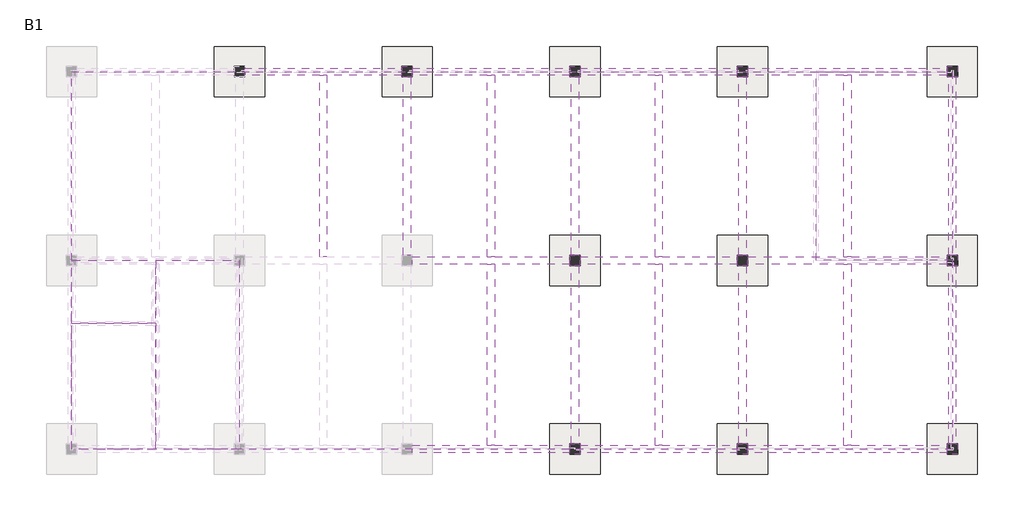
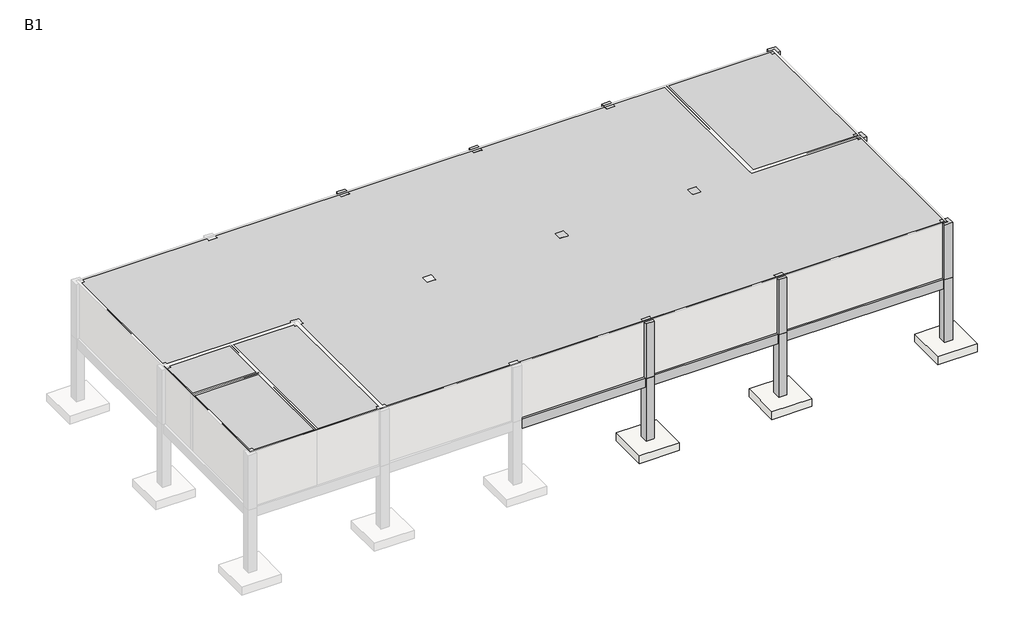
# One storey, part 2 of 2: 24 beams, 21 columns, 11 slabs, 5 proxies.
"""IFC4 building model written with IfcOpenShell, lengths in millimetres."""

import ifcopenshell
import ifcopenshell.guid

model = None  # the IFC model being written
_history = None  # IfcOwnerHistory: only IFC2X3 demands one
_inside = {}  # id of a spatial element -> (the spatial element, [elements in it])
_under = {}  # id of a project, library or spatial element -> (it, [spatial elements below it])
_declared = {}  # id of a project -> (the project, [libraries it declares])
_typed = {}  # id of a type object -> (the type object, [elements of that type])
_made_of = {}  # id of a material, layer set ... -> (it, [elements and type objects made of it])


def new_model(schema):
    """Start an empty IFC model of exactly this schema.

    Asked for "IFC4X3", IfcOpenShell would pick the latest addendum, in which some entities
    have other attributes; the version numbers below select the first issue.
    IFC2X3 requires an IfcOwnerHistory on every rooted entity: one is made here for all.
    """
    global model, _history
    if schema == "IFC4X3":
        model = ifcopenshell.file(schema_version=(4, 3, 0, 0))
    else:
        model = ifcopenshell.file(schema=schema)
    _inside.clear()
    _under.clear()
    _declared.clear()
    _typed.clear()
    _made_of.clear()
    _history = None
    if model.schema == "IFC2X3":
        org = make("IfcOrganization", Name="unknown")
        user = make(
            "IfcPersonAndOrganization",
            ThePerson=make("IfcPerson", FamilyName="unknown"),
            TheOrganization=org,
        )
        app = make(
            "IfcApplication",
            ApplicationDeveloper=org,
            Version="unknown",
            ApplicationFullName="unknown",
            ApplicationIdentifier="unknown",
        )
        _history = make(
            "IfcOwnerHistory",
            OwningUser=user,
            OwningApplication=app,
            ChangeAction="ADDED",
            CreationDate=0,
        )
    return model


def make(cls, **values):
    """One entity of the class cls with the attributes given. An attribute that is None is left unset."""
    return model.create_entity(
        cls, **{name: value for name, value in values.items() if value is not None}
    )


def rooted(cls, **values):
    """An entity with a GlobalId (a new one), such as an element, a storey or a relation."""
    return make(cls, GlobalId=ifcopenshell.guid.new(), OwnerHistory=_history, **values)


def si_unit(unit_type, name, prefix=None):
    """IfcSIUnit, for example si_unit("LENGTHUNIT", "METRE", prefix="MILLI")."""
    return make("IfcSIUnit", UnitType=unit_type, Prefix=prefix, Name=name)


def assignment(units):
    """IfcUnitAssignment: the units of a project."""
    return None if units is None else make("IfcUnitAssignment", Units=units)


def point(xyz):
    """IfcCartesianPoint."""
    return None if xyz is None else make("IfcCartesianPoint", Coordinates=xyz)


def direction(xyz):
    """IfcDirection."""
    return None if xyz is None else make("IfcDirection", DirectionRatios=xyz)


def frame(location, z_axis=None, x_axis=None):
    """IfcAxis2Placement3D, a coordinate frame: its origin and axes. An axis left out is left unset."""
    return make(
        "IfcAxis2Placement3D",
        Location=point(location),
        Axis=direction(z_axis),
        RefDirection=direction(x_axis),
    )


def origin():
    """The frame at (0, 0, 0) with its axes left unset."""
    return frame((0.0, 0.0, 0.0))


def origin_with_axes():
    """The frame at (0, 0, 0) with the z axis (0, 0, 1) and the x axis (1, 0, 0) written out."""
    return frame((0.0, 0.0, 0.0), z_axis=(0.0, 0.0, 1.0), x_axis=(1.0, 0.0, 0.0))


def place(relative_to, where):
    """IfcLocalPlacement: puts the frame where relative to a parent placement (None: the world)."""
    return make(
        "IfcLocalPlacement", PlacementRelTo=relative_to, RelativePlacement=where
    )


def context(
    kind, dimensions, precision=None, world=None, true_north=None, identifier=None
):
    """IfcGeometricRepresentationContext, for example the 3D "Model" context."""
    return make(
        "IfcGeometricRepresentationContext",
        ContextIdentifier=identifier,
        ContextType=kind,
        CoordinateSpaceDimension=dimensions,
        Precision=precision,
        WorldCoordinateSystem=world,
        TrueNorth=true_north,
    )


def project(units=None, contexts=None):
    """IfcProject with its units and contexts."""
    return rooted(
        "IfcProject",
        Name="project",
        RepresentationContexts=contexts,
        UnitsInContext=assignment(units),
    )


def spatial(cls, under=None, at=None, **own):
    """A site, building, storey or space (cls), placed at a placement, below another one or the project."""
    s = rooted(cls, ObjectPlacement=at, **own)
    if under is not None:
        _under.setdefault(under.id(), (under, []))[1].append(s)
    return s


def polyline(points):
    """IfcPolyline through the points."""
    return make("IfcPolyline", Points=[point(p) for p in points])


def outline(outer, holes=None, kind="AREA"):
    """IfcArbitraryClosedProfileDef: a profile drawn as a closed curve; with holes, ...WithVoids."""
    if holes is None:
        return make("IfcArbitraryClosedProfileDef", ProfileType=kind, OuterCurve=outer)
    return make(
        "IfcArbitraryProfileDefWithVoids",
        ProfileType=kind,
        OuterCurve=outer,
        InnerCurves=holes,
    )


def extrude(swept, where, along, depth):
    """IfcExtrudedAreaSolid: the profile swept, set in the frame where, extruded along a direction by depth."""
    return make(
        "IfcExtrudedAreaSolid",
        SweptArea=swept,
        Position=where,
        ExtrudedDirection=direction(along),
        Depth=depth,
    )


def faces_of(points, faces, orient=None, outer=None):
    """IfcFace entities. A face is a list of loops; a loop is a list of indices into points, from 0.

    orient and outer hold one flag for each loop. By default every Orientation is true, the
    first loop of a face is its IfcFaceOuterBound and the others are IfcFaceBound.
    """
    made = []
    for i, loops in enumerate(faces):
        bounds = []
        for j, loop in enumerate(loops):
            is_outer = j == 0 if outer is None else outer[i][j]
            bounds.append(
                make(
                    "IfcFaceOuterBound" if is_outer else "IfcFaceBound",
                    Bound=make("IfcPolyLoop", Polygon=[points[k] for k in loop]),
                    Orientation=True if orient is None else orient[i][j],
                )
            )
        made.append(make("IfcFace", Bounds=bounds))
    return made


def faceted_brep(points, faces, orient=None, outer=None, voids=None):
    """IfcFacetedBrep: a solid bounded by flat faces; with voids (closed shells), ...WithVoids."""
    shared = [point(p) for p in points]
    hull = make("IfcClosedShell", CfsFaces=faces_of(shared, faces, orient, outer))
    if voids is None:
        return make("IfcFacetedBrep", Outer=hull)
    return make(
        "IfcFacetedBrepWithVoids",
        Outer=hull,
        Voids=[
            make(cls, CfsFaces=faces_of(shared, fs, o, b)) for cls, fs, o, b in voids
        ],
    )


def shape(context_of_items, identifier, shape_type, items):
    """IfcShapeRepresentation: the items that make up one representation, for example the "Body"."""
    return make(
        "IfcShapeRepresentation",
        ContextOfItems=context_of_items,
        RepresentationIdentifier=identifier,
        RepresentationType=shape_type,
        Items=items,
    )


def source(mapping_origin, context_of_items, identifier, shape_type, items):
    """IfcRepresentationMap: a shape defined once, which mapped items show again and again."""
    return make(
        "IfcRepresentationMap",
        MappingOrigin=mapping_origin,
        MappedRepresentation=shape(context_of_items, identifier, shape_type, items),
    )


def transform(
    local_origin,
    x_axis=None,
    y_axis=None,
    z_axis=None,
    scale=None,
    scale2=None,
    scale3=None,
    uniform=True,
):
    """IfcCartesianTransformationOperator3D, or its non-uniform kind. x_axis, y_axis, z_axis: its Axis1, 2, 3."""
    if uniform:
        return make(
            "IfcCartesianTransformationOperator3D",
            Axis1=direction(x_axis),
            Axis2=direction(y_axis),
            LocalOrigin=point(local_origin),
            Scale=scale,
            Axis3=direction(z_axis),
        )
    return make(
        "IfcCartesianTransformationOperator3DnonUniform",
        Axis1=direction(x_axis),
        Axis2=direction(y_axis),
        LocalOrigin=point(local_origin),
        Scale=scale,
        Axis3=direction(z_axis),
        Scale2=scale2,
        Scale3=scale3,
    )


def mapped(mapping_source, mapping_target):
    """IfcMappedItem: shows the shape of a source again, moved by a transform."""
    return make(
        "IfcMappedItem", MappingSource=mapping_source, MappingTarget=mapping_target
    )


def made_of(thing, what):
    """Note that an element or type object is made of a material, layer set ...; save() writes the relation."""
    if what is not None:
        _made_of.setdefault(what.id(), (what, []))[1].append(thing)
    return thing


def element(
    cls,
    number,
    at=None,
    inside=None,
    cuts=None,
    type_object=None,
    material=None,
    context=None,
    identifier="Body",
    shape_type=None,
    held_by="IfcProductDefinitionShape",
    body=None,
    shapes=None,
    **own,
):
    """One element of the class cls, such as IfcWall. Its Tag is "e" and its number.

    at: its placement. inside: the storey or other place that contains it. cuts: it is an
    opening in that element (IfcRelVoidsElement). A single representation is given by context,
    identifier, shape_type and body (its items); several are given by shapes. held_by: the class
    of the entity that holds the representations. save() writes the other relations.
    """
    e = rooted(cls, Tag="e%d" % number, ObjectPlacement=at, **own)
    if body is not None:
        shapes = [shape(context, identifier, shape_type, body)]
    if shapes is not None:
        e.Representation = make(held_by, Representations=shapes)
    if inside is not None:
        _inside.setdefault(inside.id(), (inside, []))[1].append(e)
    if cuts is not None:
        rooted(
            "IfcRelVoidsElement", RelatingBuildingElement=cuts, RelatedOpeningElement=e
        )
    if type_object is not None:
        _typed.setdefault(type_object.id(), (type_object, []))[1].append(e)
    return made_of(e, material)


def aggregate(whole, parts):
    """IfcRelAggregates: a whole, such as a stair, and the parts it consists of."""
    return rooted("IfcRelAggregates", RelatingObject=whole, RelatedObjects=parts)


def save(model, path):
    """Write the relations noted so far, then the file.

    IfcRelAggregates (storeys below a building ...), IfcRelContainedInSpatialStructure (elements
    in a storey), IfcRelDefinesByType, IfcRelAssociatesMaterial and IfcRelDeclares: one each for
    every whole, place, type object, material and project.
    """
    for whole, parts in _under.values():
        aggregate(whole, parts)
    for where, things in _inside.values():
        rooted(
            "IfcRelContainedInSpatialStructure",
            RelatedElements=things,
            RelatingStructure=where,
        )
    for kind, things in _typed.values():
        rooted("IfcRelDefinesByType", RelatedObjects=things, RelatingType=kind)
    for what, things in _made_of.values():
        rooted("IfcRelAssociatesMaterial", RelatedObjects=things, RelatingMaterial=what)
    for by, libraries in _declared.values():
        rooted("IfcRelDeclares", RelatingContext=by, RelatedDefinitions=libraries)
    model.write(path)


def generic_models_bb515c93(model_context):
    return source(origin(), model_context, "Body", "SweptSolid", [
        extrude(outline(polyline([(9000.0, 21000.0), (9000.0, -21000.0), (-9000.0, -21000.0), (-9000.0, 21000.0), (9000.0, 21000.0)])), origin_with_axes(), (0.0, 0.0, 1.0), 3500.0),
    ])


def generic_models_5926095e(model_context):
    return source(origin(), model_context, "Body", "SweptSolid", [
        extrude(outline(polyline([(3250.0, 4500.0), (3250.0, -4500.0), (-3250.0, -4500.0), (-3250.0, 4500.0), (3250.0, 4500.0)])), origin_with_axes(), (0.0, 0.0, 1.0), 3500.0),
    ])


def generic_models_0b067365(model_context):
    return source(origin(), model_context, "Body", "SweptSolid", [
        extrude(outline(polyline([(2000.0, 4500.0), (2000.0, -4500.0), (-2000.0, -4500.0), (-2000.0, 4500.0), (2000.0, 4500.0)])), origin_with_axes(), (0.0, 0.0, 1.0), 3500.0),
    ])


def generic_models_4c644d41(model_context):
    return source(origin(), model_context, "Body", "SweptSolid", [
        extrude(outline(polyline([(2000.0, 1500.0), (2000.0, -1500.0), (-2000.0, -1500.0), (-2000.0, 1500.0), (2000.0, 1500.0)])), origin_with_axes(), (0.0, 0.0, 1.0), 3500.0),
    ])


def generic_models_c89eb543(model_context):
    return source(origin(), model_context, "Body", "SweptSolid", [
        extrude(outline(polyline([(2000.0, 3000.0), (2000.0, -3000.0), (-2000.0, -3000.0), (-2000.0, 3000.0), (2000.0, 3000.0)])), origin_with_axes(), (0.0, 0.0, 1.0), 3500.0),
    ])


def ft112_footing_rectangular_ft112_2400x2400x500_5fe39465(model_context):
    return source(origin(), model_context, "Body", "SweptSolid", [
        extrude(outline(polyline([(1200.0, 1200.0), (1200.0, -1200.0), (-1200.0, -1200.0), (-1200.0, 1200.0), (1200.0, 1200.0)])), frame((0.0, 0.0, -500.0), z_axis=(0.0, 0.0, 1.0), x_axis=(1.0, 0.0, 0.0)), (0.0, 0.0, 1.0), 500.0),
    ])


model = new_model("IFC4")

# Units and contexts
model_context = context("Model", 3, world=origin())
ifc_project = project(units=[si_unit("LENGTHUNIT", "METRE", prefix="MILLI")], contexts=[model_context])

# Site, building, storey
site = spatial("IfcSite", under=ifc_project)
building = spatial("IfcBuilding", under=site)
storey = spatial("IfcBuildingStorey", under=building, Name="B1", Elevation=-4000.0)

# Beams
placement = place(None, origin())
element("IfcBeam", 1, ObjectType="Concrete-Rectangular-Beam : BM111_400x500_RG1", at=placement, inside=storey, context=model_context, shape_type="SweptSolid", body=[
    extrude(outline(polyline([(57634.6521483, 173098.8614395), (57284.6521483, 173098.8614395), (57284.6521483, 181748.8614395), (57634.6521483, 181748.8614395), (57634.6521483, 173098.8614395)])), frame((0.0, 0.0, -600.0), z_axis=(0.0, 0.0, 1.0), x_axis=(1.0, 0.0, 0.0)), (0.0, 0.0, 1.0), 600.0),
])
element("IfcBeam", 2, ObjectType="Concrete-Rectangular-Beam : BM111_400x500_RG1", at=placement, inside=storey, context=model_context, shape_type="SweptSolid", body=[
    extrude(outline(polyline([(65634.6521483, 173098.8614395), (65284.6521483, 173098.8614395), (65284.6521483, 181748.8614395), (65634.6521483, 181748.8614395), (65634.6521483, 173098.8614395)])), frame((0.0, 0.0, -600.0), z_axis=(0.0, 0.0, 1.0), x_axis=(1.0, 0.0, 0.0)), (0.0, 0.0, 1.0), 600.0),
])
element("IfcBeam", 3, ObjectType="Concrete-Rectangular-Beam : BM111_400x500_RG1", at=placement, inside=storey, context=model_context, shape_type="SweptSolid", body=[
    extrude(outline(polyline([(65284.6521483, 172748.8614395), (65634.6521483, 172748.8614395), (65634.6521483, 164098.8614395), (65284.6521483, 164098.8614395), (65284.6521483, 172748.8614395)])), frame((0.0, 0.0, -600.0), z_axis=(0.0, 0.0, 1.0), x_axis=(1.0, 0.0, 0.0)), (0.0, 0.0, 1.0), 600.0),
])
element("IfcBeam", 4, ObjectType="Concrete-Rectangular-Beam : BM111_400x500_RG1", at=placement, inside=storey, context=model_context, shape_type="SweptSolid", body=[
    extrude(outline(polyline([(73634.6521483, 173098.8614395), (73284.6521483, 173098.8614395), (73284.6521483, 181748.8614395), (73634.6521483, 181748.8614395), (73634.6521483, 173098.8614395)])), frame((0.0, 0.0, -600.0), z_axis=(0.0, 0.0, 1.0), x_axis=(1.0, 0.0, 0.0)), (0.0, 0.0, 1.0), 600.0),
])
element("IfcBeam", 5, ObjectType="Concrete-Rectangular-Beam : BM111_400x500_RG1", at=placement, inside=storey, context=model_context, shape_type="SweptSolid", body=[
    extrude(outline(polyline([(73284.6521483, 172748.8614395), (73634.6521483, 172748.8614395), (73634.6521483, 164098.8614395), (73284.6521483, 164098.8614395), (73284.6521483, 172748.8614395)])), frame((0.0, 0.0, -600.0), z_axis=(0.0, 0.0, 1.0), x_axis=(1.0, 0.0, 0.0)), (0.0, 0.0, 1.0), 600.0),
])
element("IfcBeam", 6, ObjectType="Concrete-Rectangular-Beam : BM111_400x500_RG1", at=placement, inside=storey, context=model_context, shape_type="SweptSolid", body=[
    extrude(outline(polyline([(82634.6521483, 173098.8614395), (82284.6521483, 173098.8614395), (82284.6521483, 181748.8614395), (82634.6521483, 181748.8614395), (82634.6521483, 173098.8614395)])), frame((0.0, 0.0, -600.0), z_axis=(0.0, 0.0, 1.0), x_axis=(1.0, 0.0, 0.0)), (0.0, 0.0, 1.0), 600.0),
])
element("IfcBeam", 7, ObjectType="Concrete-Rectangular-Beam : BM111_400x500_RG1", at=placement, inside=storey, context=model_context, shape_type="SweptSolid", body=[
    extrude(outline(polyline([(82284.6521483, 172748.8614395), (82634.6521483, 172748.8614395), (82634.6521483, 164098.8614395), (82284.6521483, 164098.8614395), (82284.6521483, 172748.8614395)])), frame((0.0, 0.0, -600.0), z_axis=(0.0, 0.0, 1.0), x_axis=(1.0, 0.0, 0.0)), (0.0, 0.0, 1.0), 600.0),
])
element("IfcBeam", 8, ObjectType="Concrete-Rectangular-Beam : BM111_400x500_RG1", at=placement, inside=storey, context=model_context, shape_type="Brep", body=[
    faceted_brep([(53709.6521483, 182098.8614395, 0.0), (53709.6521483, 181748.8614395, 0.0), (57284.6521483, 181748.8614395, 0.0), (57634.6521483, 181748.8614395, 0.0), (61209.6521483, 181748.8614395, 0.0), (61209.6521483, 182098.8614395, 0.0), (53709.6521483, 181748.8614395, -600.0), (57284.6521483, 181748.8614395, -600.0), (57634.6521483, 181748.8614395, -600.0), (61209.6521483, 181748.8614395, -600.0), (53709.6521483, 182098.8614395, -600.0), (61209.6521483, 182098.8614395, -600.0)], [[[0, 1, 2, 3, 4, 5]], [[1, 6, 7, 8, 9, 4, 3, 2]], [[6, 10, 11, 9, 8, 7]], [[10, 0, 5, 11]], [[1, 0, 10, 6]], [[5, 4, 9, 11]]]),
])
element("IfcBeam", 9, ObjectType="Concrete-Rectangular-Beam : BM111_400x500_RG1", at=placement, inside=storey, context=model_context, shape_type="Brep", body=[
    faceted_brep([(61709.6521483, 182098.8614395, 0.0), (61709.6521483, 181748.8614395, 0.0), (65284.6521483, 181748.8614395, 0.0), (65634.6521483, 181748.8614395, 0.0), (69209.6521483, 181748.8614395, 0.0), (69209.6521483, 182098.8614395, 0.0), (61709.6521483, 181748.8614395, -600.0), (65284.6521483, 181748.8614395, -600.0), (65634.6521483, 181748.8614395, -600.0), (69209.6521483, 181748.8614395, -600.0), (61709.6521483, 182098.8614395, -600.0), (69209.6521483, 182098.8614395, -600.0)], [[[0, 1, 2, 3, 4, 5]], [[1, 6, 7, 8, 9, 4, 3, 2]], [[6, 10, 11, 9, 8, 7]], [[10, 0, 5, 11]], [[1, 0, 10, 6]], [[5, 4, 9, 11]]]),
])
element("IfcBeam", 10, ObjectType="Concrete-Rectangular-Beam : BM111_400x500_RG1", at=placement, inside=storey, context=model_context, shape_type="Brep", body=[
    faceted_brep([(69709.6521483, 182098.8614395, 0.0), (69709.6521483, 181748.8614395, 0.0), (73284.6521483, 181748.8614395, 0.0), (73634.6521483, 181748.8614395, 0.0), (77209.6521483, 181748.8614395, 0.0), (77209.6521483, 182098.8614395, 0.0), (69709.6521483, 181748.8614395, -600.0), (73284.6521483, 181748.8614395, -600.0), (73634.6521483, 181748.8614395, -600.0), (77209.6521483, 181748.8614395, -600.0), (69709.6521483, 182098.8614395, -600.0), (77209.6521483, 182098.8614395, -600.0)], [[[0, 1, 2, 3, 4, 5]], [[1, 6, 7, 8, 9, 4, 3, 2]], [[6, 10, 11, 9, 8, 7]], [[10, 0, 5, 11]], [[1, 0, 10, 6]], [[5, 4, 9, 11]]]),
])
element("IfcBeam", 11, ObjectType="Concrete-Rectangular-Beam : BM111_400x500_RG1", at=placement, inside=storey, context=model_context, shape_type="Brep", body=[
    faceted_brep([(77709.6521483, 182098.8614395, 0.0), (77709.6521483, 181748.8614395, 0.0), (82284.6521483, 181748.8614395, 0.0), (82634.6521483, 181748.8614395, 0.0), (87209.6521483, 181748.8614395, 0.0), (87209.6521483, 182098.8614395, 0.0), (77709.6521483, 181748.8614395, -600.0), (82284.6521483, 181748.8614395, -600.0), (82634.6521483, 181748.8614395, -600.0), (87209.6521483, 181748.8614395, -600.0), (77709.6521483, 182098.8614395, -600.0), (87209.6521483, 182098.8614395, -600.0)], [[[0, 1, 2, 3, 4, 5]], [[1, 6, 7, 8, 9, 4, 3, 2]], [[6, 10, 11, 9, 8, 7]], [[10, 0, 5, 11]], [[1, 0, 10, 6]], [[5, 4, 9, 11]]]),
])
element("IfcBeam", 12, ObjectType="Concrete-Rectangular-Beam : BM111_400x500_RG1", at=placement, inside=storey, context=model_context, shape_type="Brep", body=[
    faceted_brep([(61709.6521483, 173098.8614395, 0.0), (61709.6521483, 172748.8614395, 0.0), (65284.6521483, 172748.8614395, 0.0), (65634.6521483, 172748.8614395, 0.0), (69209.6521483, 172748.8614395, 0.0), (69209.6521483, 173098.8614395, 0.0), (65634.6521483, 173098.8614395, 0.0), (65284.6521483, 173098.8614395, 0.0), (61709.6521483, 172748.8614395, -600.0), (65284.6521483, 172748.8614395, -600.0), (65634.6521483, 172748.8614395, -600.0), (69209.6521483, 172748.8614395, -600.0), (61709.6521483, 173098.8614395, -600.0), (65284.6521483, 173098.8614395, -600.0), (65634.6521483, 173098.8614395, -600.0), (69209.6521483, 173098.8614395, -600.0)], [[[0, 1, 2, 3, 4, 5, 6, 7]], [[1, 8, 9, 10, 11, 4, 3, 2]], [[8, 12, 13, 14, 15, 11, 10, 9]], [[12, 0, 7, 6, 5, 15, 14, 13]], [[1, 0, 12, 8]], [[5, 4, 11, 15]]]),
])
element("IfcBeam", 13, ObjectType="Concrete-Rectangular-Beam : BM111_400x500_RG1", at=placement, inside=storey, context=model_context, shape_type="Brep", body=[
    faceted_brep([(69709.6521483, 173098.8614395, 0.0), (69709.6521483, 172748.8614395, 0.0), (73284.6521483, 172748.8614395, 0.0), (73634.6521483, 172748.8614395, 0.0), (77209.6521483, 172748.8614395, 0.0), (77209.6521483, 173098.8614395, 0.0), (73634.6521483, 173098.8614395, 0.0), (73284.6521483, 173098.8614395, 0.0), (69709.6521483, 172748.8614395, -600.0), (73284.6521483, 172748.8614395, -600.0), (73634.6521483, 172748.8614395, -600.0), (77209.6521483, 172748.8614395, -600.0), (69709.6521483, 173098.8614395, -600.0), (73284.6521483, 173098.8614395, -600.0), (73634.6521483, 173098.8614395, -600.0), (77209.6521483, 173098.8614395, -600.0)], [[[0, 1, 2, 3, 4, 5, 6, 7]], [[1, 8, 9, 10, 11, 4, 3, 2]], [[8, 12, 13, 14, 15, 11, 10, 9]], [[12, 0, 7, 6, 5, 15, 14, 13]], [[1, 0, 12, 8]], [[5, 4, 11, 15]]]),
])
element("IfcBeam", 14, ObjectType="Concrete-Rectangular-Beam : BM111_400x500_RG1", at=placement, inside=storey, context=model_context, shape_type="Brep", body=[
    faceted_brep([(77709.6521483, 173098.8614395, 0.0), (77709.6521483, 172748.8614395, 0.0), (82284.6521483, 172748.8614395, 0.0), (82634.6521483, 172748.8614395, 0.0), (87209.6521483, 172748.8614395, 0.0), (87209.6521483, 173098.8614395, 0.0), (82634.6521483, 173098.8614395, 0.0), (82284.6521483, 173098.8614395, 0.0), (77709.6521483, 172748.8614395, -600.0), (82284.6521483, 172748.8614395, -600.0), (82634.6521483, 172748.8614395, -600.0), (87209.6521483, 172748.8614395, -600.0), (77709.6521483, 173098.8614395, -600.0), (82284.6521483, 173098.8614395, -600.0), (82634.6521483, 173098.8614395, -600.0), (87209.6521483, 173098.8614395, -600.0)], [[[0, 1, 2, 3, 4, 5, 6, 7]], [[1, 8, 9, 10, 11, 4, 3, 2]], [[8, 12, 13, 14, 15, 11, 10, 9]], [[12, 0, 7, 6, 5, 15, 14, 13]], [[1, 0, 12, 8]], [[5, 4, 11, 15]]]),
])
element("IfcBeam", 15, ObjectType="Concrete-Rectangular-Beam : BM111_400x500_RG1", at=placement, inside=storey, context=model_context, shape_type="Brep", body=[
    faceted_brep([(61709.6521483, 164098.8614395, 0.0), (61709.6521483, 163748.8614395, 0.0), (69209.6521483, 163748.8614395, 0.0), (69209.6521483, 164098.8614395, 0.0), (65634.6521483, 164098.8614395, 0.0), (65284.6521483, 164098.8614395, 0.0), (61709.6521483, 163748.8614395, -600.0), (69209.6521483, 163748.8614395, -600.0), (61709.6521483, 164098.8614395, -600.0), (65284.6521483, 164098.8614395, -600.0), (65634.6521483, 164098.8614395, -600.0), (69209.6521483, 164098.8614395, -600.0)], [[[0, 1, 2, 3, 4, 5]], [[1, 6, 7, 2]], [[6, 8, 9, 10, 11, 7]], [[8, 0, 5, 4, 3, 11, 10, 9]], [[1, 0, 8, 6]], [[3, 2, 7, 11]]]),
])
element("IfcBeam", 16, ObjectType="Concrete-Rectangular-Beam : BM111_400x500_RG1", at=placement, inside=storey, context=model_context, shape_type="Brep", body=[
    faceted_brep([(69709.6521483, 164098.8614395, 0.0), (69709.6521483, 163748.8614395, 0.0), (77209.6521483, 163748.8614395, 0.0), (77209.6521483, 164098.8614395, 0.0), (73634.6521483, 164098.8614395, 0.0), (73284.6521483, 164098.8614395, 0.0), (69709.6521483, 163748.8614395, -600.0), (77209.6521483, 163748.8614395, -600.0), (69709.6521483, 164098.8614395, -600.0), (73284.6521483, 164098.8614395, -600.0), (73634.6521483, 164098.8614395, -600.0), (77209.6521483, 164098.8614395, -600.0)], [[[0, 1, 2, 3, 4, 5]], [[1, 6, 7, 2]], [[6, 8, 9, 10, 11, 7]], [[8, 0, 5, 4, 3, 11, 10, 9]], [[1, 0, 8, 6]], [[3, 2, 7, 11]]]),
])
element("IfcBeam", 17, ObjectType="Concrete-Rectangular-Beam : BM111_400x500_RG1", at=placement, inside=storey, context=model_context, shape_type="Brep", body=[
    faceted_brep([(77709.6521483, 164098.8614395, 0.0), (77709.6521483, 163748.8614395, 0.0), (87209.6521483, 163748.8614395, 0.0), (87209.6521483, 164098.8614395, 0.0), (82634.6521483, 164098.8614395, 0.0), (82284.6521483, 164098.8614395, 0.0), (77709.6521483, 163748.8614395, -600.0), (87209.6521483, 163748.8614395, -600.0), (77709.6521483, 164098.8614395, -600.0), (82284.6521483, 164098.8614395, -600.0), (82634.6521483, 164098.8614395, -600.0), (87209.6521483, 164098.8614395, -600.0)], [[[0, 1, 2, 3, 4, 5]], [[1, 6, 7, 2]], [[6, 8, 9, 10, 11, 7]], [[8, 0, 5, 4, 3, 11, 10, 9]], [[1, 0, 8, 6]], [[3, 2, 7, 11]]]),
])
element("IfcBeam", 18, ObjectType="Concrete-Rectangular-Beam : BM111_400x500_RG1", at=placement, inside=storey, context=model_context, shape_type="SweptSolid", body=[
    extrude(outline(polyline([(61284.6521483, 181673.8614395), (61634.6521483, 181673.8614395), (61634.6521483, 173173.8614395), (61284.6521483, 173173.8614395), (61284.6521483, 181673.8614395)])), frame((0.0, 0.0, -600.0), z_axis=(0.0, 0.0, 1.0), x_axis=(1.0, 0.0, 0.0)), (0.0, 0.0, 1.0), 600.0),
])
element("IfcBeam", 19, ObjectType="Concrete-Rectangular-Beam : BM111_400x500_RG1", at=placement, inside=storey, context=model_context, shape_type="SweptSolid", body=[
    extrude(outline(polyline([(69284.6521483, 181673.8614395), (69634.6521483, 181673.8614395), (69634.6521483, 173173.8614395), (69284.6521483, 173173.8614395), (69284.6521483, 181673.8614395)])), frame((0.0, 0.0, -600.0), z_axis=(0.0, 0.0, 1.0), x_axis=(1.0, 0.0, 0.0)), (0.0, 0.0, 1.0), 600.0),
])
element("IfcBeam", 20, ObjectType="Concrete-Rectangular-Beam : BM111_400x500_RG1", at=placement, inside=storey, context=model_context, shape_type="SweptSolid", body=[
    extrude(outline(polyline([(69284.6521483, 172673.8614395), (69634.6521483, 172673.8614395), (69634.6521483, 164173.8614395), (69284.6521483, 164173.8614395), (69284.6521483, 172673.8614395)])), frame((0.0, 0.0, -600.0), z_axis=(0.0, 0.0, 1.0), x_axis=(1.0, 0.0, 0.0)), (0.0, 0.0, 1.0), 600.0),
])
element("IfcBeam", 21, ObjectType="Concrete-Rectangular-Beam : BM111_400x500_RG1", at=placement, inside=storey, context=model_context, shape_type="SweptSolid", body=[
    extrude(outline(polyline([(77284.6521483, 181673.8614395), (77634.6521483, 181673.8614395), (77634.6521483, 173173.8614395), (77284.6521483, 173173.8614395), (77284.6521483, 181673.8614395)])), frame((0.0, 0.0, -600.0), z_axis=(0.0, 0.0, 1.0), x_axis=(1.0, 0.0, 0.0)), (0.0, 0.0, 1.0), 600.0),
])
element("IfcBeam", 22, ObjectType="Concrete-Rectangular-Beam : BM111_400x500_RG1", at=placement, inside=storey, context=model_context, shape_type="SweptSolid", body=[
    extrude(outline(polyline([(77284.6521483, 172673.8614395), (77634.6521483, 172673.8614395), (77634.6521483, 164173.8614395), (77284.6521483, 164173.8614395), (77284.6521483, 172673.8614395)])), frame((0.0, 0.0, -600.0), z_axis=(0.0, 0.0, 1.0), x_axis=(1.0, 0.0, 0.0)), (0.0, 0.0, 1.0), 600.0),
])
element("IfcBeam", 23, ObjectType="Concrete-Rectangular-Beam : BM111_400x500_RG1", at=placement, inside=storey, context=model_context, shape_type="SweptSolid", body=[
    extrude(outline(polyline([(87284.6521483, 181673.8614395), (87634.6521483, 181673.8614395), (87634.6521483, 173173.8614395), (87284.6521483, 173173.8614395), (87284.6521483, 181673.8614395)])), frame((0.0, 0.0, -600.0), z_axis=(0.0, 0.0, 1.0), x_axis=(1.0, 0.0, 0.0)), (0.0, 0.0, 1.0), 600.0),
])
element("IfcBeam", 24, ObjectType="Concrete-Rectangular-Beam : BM111_400x500_RG1", at=placement, inside=storey, context=model_context, shape_type="SweptSolid", body=[
    extrude(outline(polyline([(87284.6521483, 172673.8614395), (87634.6521483, 172673.8614395), (87634.6521483, 164173.8614395), (87284.6521483, 164173.8614395), (87284.6521483, 172673.8614395)])), frame((0.0, 0.0, -600.0), z_axis=(0.0, 0.0, 1.0), x_axis=(1.0, 0.0, 0.0)), (0.0, 0.0, 1.0), 600.0),
])

# Proxies
generic_models_shape = generic_models_bb515c93(model_context)
element("IfcBuildingElementProxy", 25, Name="Space Planning Box_hec : Space Planning Box_hec", ObjectType="Space Planning Box_hec : Space Planning Box_hec", at=placement, inside=storey, context=model_context, shape_type="MappedRepresentation", body=[
    mapped(generic_models_shape, transform((66459.6521483, 172923.8614395, 0.0), x_axis=(0.0, -1.0, 0.0), y_axis=(1.0, 0.0, 0.0), z_axis=(0.0, 0.0, 1.0))),
])
generic_models_2_shape = generic_models_5926095e(model_context)
element("IfcBuildingElementProxy", 26, Name="Space Planning Box_hec : Space Planning Box_hec", ObjectType="Space Planning Box_hec : Space Planning Box_hec", at=placement, inside=storey, context=model_context, shape_type="MappedRepresentation", body=[
    mapped(generic_models_2_shape, transform((84209.6521483, 177423.8614395, 0.0), x_axis=(1.0, 0.0, 0.0), y_axis=(0.0, 1.0, 0.0), z_axis=(0.0, 0.0, 1.0))),
])
generic_models_3_shape = generic_models_0b067365(model_context)
element("IfcBuildingElementProxy", 27, Name="Space Planning Box_hec : Space Planning Box_hec", ObjectType="Space Planning Box_hec : Space Planning Box_hec", at=placement, inside=storey, context=model_context, shape_type="MappedRepresentation", body=[
    mapped(generic_models_3_shape, transform((51459.6521483, 168423.8614395, 0.0), x_axis=(1.0, 0.0, 0.0), y_axis=(0.0, 1.0, 0.0), z_axis=(0.0, 0.0, 1.0))),
])
generic_models_4_shape = generic_models_4c644d41(model_context)
element("IfcBuildingElementProxy", 28, Name="Space Planning Box_hec : Space Planning Box_hec", ObjectType="Space Planning Box_hec : Space Planning Box_hec", at=placement, inside=storey, context=model_context, shape_type="MappedRepresentation", body=[
    mapped(generic_models_4_shape, transform((47459.6521483, 171423.8614395, 0.0), x_axis=(1.0, 0.0, 0.0), y_axis=(0.0, 1.0, 0.0), z_axis=(0.0, 0.0, 1.0))),
])
generic_models_5_shape = generic_models_c89eb543(model_context)
element("IfcBuildingElementProxy", 29, Name="Space Planning Box_hec : Space Planning Box_hec", ObjectType="Space Planning Box_hec : Space Planning Box_hec", at=placement, inside=storey, context=model_context, shape_type="MappedRepresentation", body=[
    mapped(generic_models_5_shape, transform((47459.6521483, 166923.8614395, 0.0), x_axis=(1.0, 0.0, 0.0), y_axis=(0.0, 1.0, 0.0), z_axis=(0.0, 0.0, 1.0))),
])

# Columns
element("IfcColumn", 30, ObjectType="Concrete-Rectangular-Column : CL111_500x500", at=placement, inside=storey, context=model_context, shape_type="Brep", body=[
    faceted_brep([(61709.6521483, 182173.8614395, 0.0), (61709.6521483, 181673.8614395, 0.0), (61209.6521483, 181673.8614395, 0.0), (61209.6521483, 182173.8614395, 0.0), (61709.6521483, 182173.8614395, 3500.0), (61709.6521483, 182098.8614395, 3500.0), (61709.6521483, 181748.8614395, 3500.0), (61709.6521483, 181673.8614395, 3500.0), (61634.6521483, 181673.8614395, 3500.0), (61284.6521483, 181673.8614395, 3500.0), (61209.6521483, 181673.8614395, 3500.0), (61209.6521483, 181748.8614395, 3500.0), (61209.6521483, 182098.8614395, 3500.0), (61209.6521483, 182173.8614395, 3500.0)], [[[0, 1, 2, 3]], [[4, 5, 6, 7, 1, 0]], [[7, 8, 9, 10, 2, 1]], [[10, 11, 12, 13, 3, 2]], [[13, 4, 0, 3]], [[4, 13, 12, 11, 10, 9, 8, 7, 6, 5]]]),
])
element("IfcColumn", 31, ObjectType="Concrete-Rectangular-Column : CL111_500x500", at=placement, inside=storey, context=model_context, shape_type="Brep", body=[
    faceted_brep([(69709.6521483, 182173.8614395, 0.0), (69709.6521483, 181673.8614395, 0.0), (69209.6521483, 181673.8614395, 0.0), (69209.6521483, 182173.8614395, 0.0), (69709.6521483, 182173.8614395, 3500.0), (69709.6521483, 182098.8614395, 3500.0), (69709.6521483, 181748.8614395, 3500.0), (69709.6521483, 181673.8614395, 3500.0), (69634.6521483, 181673.8614395, 3500.0), (69284.6521483, 181673.8614395, 3500.0), (69209.6521483, 181673.8614395, 3500.0), (69209.6521483, 181748.8614395, 3500.0), (69209.6521483, 182098.8614395, 3500.0), (69209.6521483, 182173.8614395, 3500.0)], [[[0, 1, 2, 3]], [[4, 5, 6, 7, 1, 0]], [[7, 8, 9, 10, 2, 1]], [[10, 11, 12, 13, 3, 2]], [[13, 4, 0, 3]], [[4, 13, 12, 11, 10, 9, 8, 7, 6, 5]]]),
])
element("IfcColumn", 32, ObjectType="Concrete-Rectangular-Column : CL111_500x500", at=placement, inside=storey, context=model_context, shape_type="Brep", body=[
    faceted_brep([(77709.6521483, 182173.8614395, 0.0), (77709.6521483, 181673.8614395, 0.0), (77209.6521483, 181673.8614395, 0.0), (77209.6521483, 182173.8614395, 0.0), (77709.6521483, 182173.8614395, 3500.0), (77709.6521483, 182098.8614395, 3500.0), (77709.6521483, 181748.8614395, 3500.0), (77709.6521483, 181673.8614395, 3500.0), (77634.6521483, 181673.8614395, 3500.0), (77284.6521483, 181673.8614395, 3500.0), (77209.6521483, 181673.8614395, 3500.0), (77209.6521483, 181748.8614395, 3500.0), (77209.6521483, 182098.8614395, 3500.0), (77209.6521483, 182173.8614395, 3500.0)], [[[0, 1, 2, 3]], [[4, 5, 6, 7, 1, 0]], [[7, 8, 9, 10, 2, 1]], [[10, 11, 12, 13, 3, 2]], [[13, 4, 0, 3]], [[4, 13, 12, 11, 10, 9, 8, 7, 6, 5]]]),
])
element("IfcColumn", 33, ObjectType="Concrete-Rectangular-Column : CL111_500x500", at=placement, inside=storey, context=model_context, shape_type="Brep", body=[
    faceted_brep([(87709.6521483, 182173.8614395, 0.0), (87709.6521483, 181673.8614395, 0.0), (87209.6521483, 181673.8614395, 0.0), (87209.6521483, 182173.8614395, 0.0), (87709.6521483, 182173.8614395, 3500.0), (87709.6521483, 181673.8614395, 3500.0), (87634.6521483, 181673.8614395, 3500.0), (87284.6521483, 181673.8614395, 3500.0), (87209.6521483, 181673.8614395, 3500.0), (87209.6521483, 181748.8614395, 3500.0), (87209.6521483, 182098.8614395, 3500.0), (87209.6521483, 182173.8614395, 3500.0)], [[[0, 1, 2, 3]], [[4, 5, 1, 0]], [[5, 6, 7, 8, 2, 1]], [[8, 9, 10, 11, 3, 2]], [[11, 4, 0, 3]], [[4, 11, 10, 9, 8, 7, 6, 5]]]),
])
element("IfcColumn", 34, ObjectType="Concrete-Rectangular-Column : CL111_500x500", at=placement, inside=storey, context=model_context, shape_type="Brep", body=[
    faceted_brep([(69709.6521483, 173173.8614395, 0.0), (69709.6521483, 172673.8614395, 0.0), (69209.6521483, 172673.8614395, 0.0), (69209.6521483, 173173.8614395, 0.0), (69709.6521483, 173173.8614395, 3500.0), (69709.6521483, 173098.8614395, 3500.0), (69709.6521483, 172748.8614395, 3500.0), (69709.6521483, 172673.8614395, 3500.0), (69634.6521483, 172673.8614395, 3500.0), (69284.6521483, 172673.8614395, 3500.0), (69209.6521483, 172673.8614395, 3500.0), (69209.6521483, 172748.8614395, 3500.0), (69209.6521483, 173098.8614395, 3500.0), (69209.6521483, 173173.8614395, 3500.0), (69284.6521483, 173173.8614395, 3500.0), (69634.6521483, 173173.8614395, 3500.0)], [[[0, 1, 2, 3]], [[4, 5, 6, 7, 1, 0]], [[7, 8, 9, 10, 2, 1]], [[10, 11, 12, 13, 3, 2]], [[13, 14, 15, 4, 0, 3]], [[4, 15, 14, 13, 12, 11, 10, 9, 8, 7, 6, 5]]]),
])
element("IfcColumn", 35, ObjectType="Concrete-Rectangular-Column : CL111_500x500", at=placement, inside=storey, context=model_context, shape_type="Brep", body=[
    faceted_brep([(77709.6521483, 173173.8614395, 0.0), (77709.6521483, 172673.8614395, 0.0), (77209.6521483, 172673.8614395, 0.0), (77209.6521483, 173173.8614395, 0.0), (77709.6521483, 173173.8614395, 3500.0), (77709.6521483, 173098.8614395, 3500.0), (77709.6521483, 172748.8614395, 3500.0), (77709.6521483, 172673.8614395, 3500.0), (77634.6521483, 172673.8614395, 3500.0), (77284.6521483, 172673.8614395, 3500.0), (77209.6521483, 172673.8614395, 3500.0), (77209.6521483, 172748.8614395, 3500.0), (77209.6521483, 173098.8614395, 3500.0), (77209.6521483, 173173.8614395, 3500.0), (77284.6521483, 173173.8614395, 3500.0), (77634.6521483, 173173.8614395, 3500.0)], [[[0, 1, 2, 3]], [[4, 5, 6, 7, 1, 0]], [[7, 8, 9, 10, 2, 1]], [[10, 11, 12, 13, 3, 2]], [[13, 14, 15, 4, 0, 3]], [[4, 15, 14, 13, 12, 11, 10, 9, 8, 7, 6, 5]]]),
])
element("IfcColumn", 36, ObjectType="Concrete-Rectangular-Column : CL111_500x500", at=placement, inside=storey, context=model_context, shape_type="Brep", body=[
    faceted_brep([(87709.6521483, 173173.8614395, 0.0), (87709.6521483, 172673.8614395, 0.0), (87209.6521483, 172673.8614395, 0.0), (87209.6521483, 173173.8614395, 0.0), (87709.6521483, 173173.8614395, 3500.0), (87709.6521483, 172673.8614395, 3500.0), (87634.6521483, 172673.8614395, 3500.0), (87284.6521483, 172673.8614395, 3500.0), (87209.6521483, 172673.8614395, 3500.0), (87209.6521483, 172748.8614395, 3500.0), (87209.6521483, 173098.8614395, 3500.0), (87209.6521483, 173173.8614395, 3500.0), (87284.6521483, 173173.8614395, 3500.0), (87634.6521483, 173173.8614395, 3500.0)], [[[0, 1, 2, 3]], [[4, 5, 1, 0]], [[5, 6, 7, 8, 2, 1]], [[8, 9, 10, 11, 3, 2]], [[11, 12, 13, 4, 0, 3]], [[4, 13, 12, 11, 10, 9, 8, 7, 6, 5]]]),
])
element("IfcColumn", 37, ObjectType="Concrete-Rectangular-Column : CL111_500x500", at=placement, inside=storey, context=model_context, shape_type="Brep", body=[
    faceted_brep([(69709.6521483, 164173.8614395, 0.0), (69709.6521483, 163673.8614395, 0.0), (69209.6521483, 163673.8614395, 0.0), (69209.6521483, 164173.8614395, 0.0), (69709.6521483, 164173.8614395, 3500.0), (69709.6521483, 164098.8614395, 3500.0), (69709.6521483, 163748.8614395, 3500.0), (69709.6521483, 163673.8614395, 3500.0), (69209.6521483, 163673.8614395, 3500.0), (69209.6521483, 163748.8614395, 3500.0), (69209.6521483, 164098.8614395, 3500.0), (69209.6521483, 164173.8614395, 3500.0), (69284.6521483, 164173.8614395, 3500.0), (69634.6521483, 164173.8614395, 3500.0)], [[[0, 1, 2, 3]], [[4, 5, 6, 7, 1, 0]], [[7, 8, 2, 1]], [[8, 9, 10, 11, 3, 2]], [[11, 12, 13, 4, 0, 3]], [[4, 13, 12, 11, 10, 9, 8, 7, 6, 5]]]),
])
element("IfcColumn", 38, ObjectType="Concrete-Rectangular-Column : CL111_500x500", at=placement, inside=storey, context=model_context, shape_type="Brep", body=[
    faceted_brep([(77709.6521483, 164173.8614395, 0.0), (77709.6521483, 163673.8614395, 0.0), (77209.6521483, 163673.8614395, 0.0), (77209.6521483, 164173.8614395, 0.0), (77709.6521483, 164173.8614395, 3500.0), (77709.6521483, 164098.8614395, 3500.0), (77709.6521483, 163748.8614395, 3500.0), (77709.6521483, 163673.8614395, 3500.0), (77209.6521483, 163673.8614395, 3500.0), (77209.6521483, 163748.8614395, 3500.0), (77209.6521483, 164098.8614395, 3500.0), (77209.6521483, 164173.8614395, 3500.0), (77284.6521483, 164173.8614395, 3500.0), (77634.6521483, 164173.8614395, 3500.0)], [[[0, 1, 2, 3]], [[4, 5, 6, 7, 1, 0]], [[7, 8, 2, 1]], [[8, 9, 10, 11, 3, 2]], [[11, 12, 13, 4, 0, 3]], [[4, 13, 12, 11, 10, 9, 8, 7, 6, 5]]]),
])
element("IfcColumn", 39, ObjectType="Concrete-Rectangular-Column : CL111_500x500", at=placement, inside=storey, context=model_context, shape_type="Brep", body=[
    faceted_brep([(87709.6521483, 164173.8614395, 0.0), (87709.6521483, 163673.8614395, 0.0), (87209.6521483, 163673.8614395, 0.0), (87209.6521483, 164173.8614395, 0.0), (87709.6521483, 164173.8614395, 3500.0), (87709.6521483, 163673.8614395, 3500.0), (87209.6521483, 163673.8614395, 3500.0), (87209.6521483, 163748.8614395, 3500.0), (87209.6521483, 164098.8614395, 3500.0), (87209.6521483, 164173.8614395, 3500.0), (87284.6521483, 164173.8614395, 3500.0), (87634.6521483, 164173.8614395, 3500.0)], [[[0, 1, 2, 3]], [[4, 5, 1, 0]], [[5, 6, 2, 1]], [[6, 7, 8, 9, 3, 2]], [[9, 10, 11, 4, 0, 3]], [[4, 11, 10, 9, 8, 7, 6, 5]]]),
])
element("IfcColumn", 40, ObjectType="Concrete-Rectangular-Column : CL111_500x500", at=placement, inside=storey, context=model_context, shape_type="Brep", body=[
    faceted_brep([(53709.6521483, 182173.8614395, -4000.0), (53709.6521483, 181673.8614395, -4000.0), (53209.6521483, 181673.8614395, -4000.0), (53209.6521483, 182173.8614395, -4000.0), (53709.6521483, 182173.8614395, 0.0), (53709.6521483, 182098.8614395, 0.0), (53709.6521483, 181748.8614395, 0.0), (53709.6521483, 181673.8614395, 0.0), (53634.6521483, 181673.8614395, 0.0), (53284.6521483, 181673.8614395, 0.0), (53209.6521483, 181673.8614395, 0.0), (53209.6521483, 181748.8614395, 0.0), (53209.6521483, 182098.8614395, 0.0), (53209.6521483, 182173.8614395, 0.0)], [[[0, 1, 2, 3]], [[4, 5, 6, 7, 1, 0]], [[7, 8, 9, 10, 2, 1]], [[10, 11, 12, 13, 3, 2]], [[13, 4, 0, 3]], [[4, 13, 12, 11, 10, 9, 8, 7, 6, 5]]]),
])
element("IfcColumn", 41, ObjectType="Concrete-Rectangular-Column : CL111_500x500", at=placement, inside=storey, context=model_context, shape_type="Brep", body=[
    faceted_brep([(61709.6521483, 182173.8614395, -4000.0), (61709.6521483, 181673.8614395, -4000.0), (61209.6521483, 181673.8614395, -4000.0), (61209.6521483, 182173.8614395, -4000.0), (61709.6521483, 182173.8614395, 0.0), (61709.6521483, 182098.8614395, 0.0), (61709.6521483, 181748.8614395, 0.0), (61709.6521483, 181673.8614395, 0.0), (61634.6521483, 181673.8614395, 0.0), (61284.6521483, 181673.8614395, 0.0), (61209.6521483, 181673.8614395, 0.0), (61209.6521483, 181748.8614395, 0.0), (61209.6521483, 182098.8614395, 0.0), (61209.6521483, 182173.8614395, 0.0)], [[[0, 1, 2, 3]], [[4, 5, 6, 7, 1, 0]], [[7, 8, 9, 10, 2, 1]], [[10, 11, 12, 13, 3, 2]], [[13, 4, 0, 3]], [[4, 13, 12, 11, 10, 9, 8, 7, 6, 5]]]),
])
element("IfcColumn", 42, ObjectType="Concrete-Rectangular-Column : CL111_500x500", at=placement, inside=storey, context=model_context, shape_type="Brep", body=[
    faceted_brep([(69709.6521483, 182173.8614395, -4000.0), (69709.6521483, 181673.8614395, -4000.0), (69209.6521483, 181673.8614395, -4000.0), (69209.6521483, 182173.8614395, -4000.0), (69709.6521483, 182173.8614395, 0.0), (69709.6521483, 182098.8614395, 0.0), (69709.6521483, 181748.8614395, 0.0), (69709.6521483, 181673.8614395, 0.0), (69634.6521483, 181673.8614395, 0.0), (69284.6521483, 181673.8614395, 0.0), (69209.6521483, 181673.8614395, 0.0), (69209.6521483, 181748.8614395, 0.0), (69209.6521483, 182098.8614395, 0.0), (69209.6521483, 182173.8614395, 0.0)], [[[0, 1, 2, 3]], [[4, 5, 6, 7, 1, 0]], [[7, 8, 9, 10, 2, 1]], [[10, 11, 12, 13, 3, 2]], [[13, 4, 0, 3]], [[4, 13, 12, 11, 10, 9, 8, 7, 6, 5]]]),
])
element("IfcColumn", 43, ObjectType="Concrete-Rectangular-Column : CL111_500x500", at=placement, inside=storey, context=model_context, shape_type="Brep", body=[
    faceted_brep([(77709.6521483, 182173.8614395, -4000.0), (77709.6521483, 181673.8614395, -4000.0), (77209.6521483, 181673.8614395, -4000.0), (77209.6521483, 182173.8614395, -4000.0), (77709.6521483, 182173.8614395, 0.0), (77709.6521483, 182098.8614395, 0.0), (77709.6521483, 181748.8614395, 0.0), (77709.6521483, 181673.8614395, 0.0), (77634.6521483, 181673.8614395, 0.0), (77284.6521483, 181673.8614395, 0.0), (77209.6521483, 181673.8614395, 0.0), (77209.6521483, 181748.8614395, 0.0), (77209.6521483, 182098.8614395, 0.0), (77209.6521483, 182173.8614395, 0.0)], [[[0, 1, 2, 3]], [[4, 5, 6, 7, 1, 0]], [[7, 8, 9, 10, 2, 1]], [[10, 11, 12, 13, 3, 2]], [[13, 4, 0, 3]], [[4, 13, 12, 11, 10, 9, 8, 7, 6, 5]]]),
])
element("IfcColumn", 44, ObjectType="Concrete-Rectangular-Column : CL111_500x500", at=placement, inside=storey, context=model_context, shape_type="Brep", body=[
    faceted_brep([(87709.6521483, 182173.8614395, -4000.0), (87709.6521483, 181673.8614395, -4000.0), (87209.6521483, 181673.8614395, -4000.0), (87209.6521483, 182173.8614395, -4000.0), (87709.6521483, 182173.8614395, 0.0), (87709.6521483, 181673.8614395, 0.0), (87634.6521483, 181673.8614395, 0.0), (87284.6521483, 181673.8614395, 0.0), (87209.6521483, 181673.8614395, 0.0), (87209.6521483, 181748.8614395, 0.0), (87209.6521483, 182098.8614395, 0.0), (87209.6521483, 182173.8614395, 0.0)], [[[0, 1, 2, 3]], [[4, 5, 1, 0]], [[5, 6, 7, 8, 2, 1]], [[8, 9, 10, 11, 3, 2]], [[11, 4, 0, 3]], [[4, 11, 10, 9, 8, 7, 6, 5]]]),
])
element("IfcColumn", 45, ObjectType="Concrete-Rectangular-Column : CL111_500x500", at=placement, inside=storey, context=model_context, shape_type="Brep", body=[
    faceted_brep([(69709.6521483, 173173.8614395, -4000.0), (69709.6521483, 172673.8614395, -4000.0), (69209.6521483, 172673.8614395, -4000.0), (69209.6521483, 173173.8614395, -4000.0), (69709.6521483, 173173.8614395, 0.0), (69709.6521483, 173098.8614395, 0.0), (69709.6521483, 172748.8614395, 0.0), (69709.6521483, 172673.8614395, 0.0), (69634.6521483, 172673.8614395, 0.0), (69284.6521483, 172673.8614395, 0.0), (69209.6521483, 172673.8614395, 0.0), (69209.6521483, 172748.8614395, 0.0), (69209.6521483, 173098.8614395, 0.0), (69209.6521483, 173173.8614395, 0.0), (69284.6521483, 173173.8614395, 0.0), (69634.6521483, 173173.8614395, 0.0)], [[[0, 1, 2, 3]], [[4, 5, 6, 7, 1, 0]], [[7, 8, 9, 10, 2, 1]], [[10, 11, 12, 13, 3, 2]], [[13, 14, 15, 4, 0, 3]], [[4, 15, 14, 13, 12, 11, 10, 9, 8, 7, 6, 5]]]),
])
element("IfcColumn", 46, ObjectType="Concrete-Rectangular-Column : CL111_500x500", at=placement, inside=storey, context=model_context, shape_type="Brep", body=[
    faceted_brep([(77709.6521483, 173173.8614395, -4000.0), (77709.6521483, 172673.8614395, -4000.0), (77209.6521483, 172673.8614395, -4000.0), (77209.6521483, 173173.8614395, -4000.0), (77709.6521483, 173173.8614395, 0.0), (77709.6521483, 173098.8614395, 0.0), (77709.6521483, 172748.8614395, 0.0), (77709.6521483, 172673.8614395, 0.0), (77634.6521483, 172673.8614395, 0.0), (77284.6521483, 172673.8614395, 0.0), (77209.6521483, 172673.8614395, 0.0), (77209.6521483, 172748.8614395, 0.0), (77209.6521483, 173098.8614395, 0.0), (77209.6521483, 173173.8614395, 0.0), (77284.6521483, 173173.8614395, 0.0), (77634.6521483, 173173.8614395, 0.0)], [[[0, 1, 2, 3]], [[4, 5, 6, 7, 1, 0]], [[7, 8, 9, 10, 2, 1]], [[10, 11, 12, 13, 3, 2]], [[13, 14, 15, 4, 0, 3]], [[4, 15, 14, 13, 12, 11, 10, 9, 8, 7, 6, 5]]]),
])
element("IfcColumn", 47, ObjectType="Concrete-Rectangular-Column : CL111_500x500", at=placement, inside=storey, context=model_context, shape_type="Brep", body=[
    faceted_brep([(87709.6521483, 173173.8614395, -4000.0), (87709.6521483, 172673.8614395, -4000.0), (87209.6521483, 172673.8614395, -4000.0), (87209.6521483, 173173.8614395, -4000.0), (87709.6521483, 173173.8614395, 0.0), (87709.6521483, 172673.8614395, 0.0), (87634.6521483, 172673.8614395, 0.0), (87284.6521483, 172673.8614395, 0.0), (87209.6521483, 172673.8614395, 0.0), (87209.6521483, 172748.8614395, 0.0), (87209.6521483, 173098.8614395, 0.0), (87209.6521483, 173173.8614395, 0.0), (87284.6521483, 173173.8614395, 0.0), (87634.6521483, 173173.8614395, 0.0)], [[[0, 1, 2, 3]], [[4, 5, 1, 0]], [[5, 6, 7, 8, 2, 1]], [[8, 9, 10, 11, 3, 2]], [[11, 12, 13, 4, 0, 3]], [[4, 13, 12, 11, 10, 9, 8, 7, 6, 5]]]),
])
element("IfcColumn", 48, ObjectType="Concrete-Rectangular-Column : CL111_500x500", at=placement, inside=storey, context=model_context, shape_type="Brep", body=[
    faceted_brep([(69709.6521483, 164173.8614395, -4000.0), (69709.6521483, 163673.8614395, -4000.0), (69209.6521483, 163673.8614395, -4000.0), (69209.6521483, 164173.8614395, -4000.0), (69709.6521483, 164173.8614395, 0.0), (69709.6521483, 164098.8614395, 0.0), (69709.6521483, 163748.8614395, 0.0), (69709.6521483, 163673.8614395, 0.0), (69209.6521483, 163673.8614395, 0.0), (69209.6521483, 163748.8614395, 0.0), (69209.6521483, 164098.8614395, 0.0), (69209.6521483, 164173.8614395, 0.0), (69284.6521483, 164173.8614395, 0.0), (69634.6521483, 164173.8614395, 0.0)], [[[0, 1, 2, 3]], [[4, 5, 6, 7, 1, 0]], [[7, 8, 2, 1]], [[8, 9, 10, 11, 3, 2]], [[11, 12, 13, 4, 0, 3]], [[4, 13, 12, 11, 10, 9, 8, 7, 6, 5]]]),
])
element("IfcColumn", 49, ObjectType="Concrete-Rectangular-Column : CL111_500x500", at=placement, inside=storey, context=model_context, shape_type="Brep", body=[
    faceted_brep([(77709.6521483, 164173.8614395, -4000.0), (77709.6521483, 163673.8614395, -4000.0), (77209.6521483, 163673.8614395, -4000.0), (77209.6521483, 164173.8614395, -4000.0), (77709.6521483, 164173.8614395, 0.0), (77709.6521483, 164098.8614395, 0.0), (77709.6521483, 163748.8614395, 0.0), (77709.6521483, 163673.8614395, 0.0), (77209.6521483, 163673.8614395, 0.0), (77209.6521483, 163748.8614395, 0.0), (77209.6521483, 164098.8614395, 0.0), (77209.6521483, 164173.8614395, 0.0), (77284.6521483, 164173.8614395, 0.0), (77634.6521483, 164173.8614395, 0.0)], [[[0, 1, 2, 3]], [[4, 5, 6, 7, 1, 0]], [[7, 8, 2, 1]], [[8, 9, 10, 11, 3, 2]], [[11, 12, 13, 4, 0, 3]], [[4, 13, 12, 11, 10, 9, 8, 7, 6, 5]]]),
])
element("IfcColumn", 50, ObjectType="Concrete-Rectangular-Column : CL111_500x500", at=placement, inside=storey, context=model_context, shape_type="Brep", body=[
    faceted_brep([(87709.6521483, 164173.8614395, -4000.0), (87709.6521483, 163673.8614395, -4000.0), (87209.6521483, 163673.8614395, -4000.0), (87209.6521483, 164173.8614395, -4000.0), (87709.6521483, 164173.8614395, 0.0), (87709.6521483, 163673.8614395, 0.0), (87209.6521483, 163673.8614395, 0.0), (87209.6521483, 163748.8614395, 0.0), (87209.6521483, 164098.8614395, 0.0), (87209.6521483, 164173.8614395, 0.0), (87284.6521483, 164173.8614395, 0.0), (87634.6521483, 164173.8614395, 0.0)], [[[0, 1, 2, 3]], [[4, 5, 1, 0]], [[5, 6, 2, 1]], [[6, 7, 8, 9, 3, 2]], [[9, 10, 11, 4, 0, 3]], [[4, 11, 10, 9, 8, 7, 6, 5]]]),
])

# Slabs
ft112_footing_rectangular_ft112_2400x2400x500_shape = ft112_footing_rectangular_ft112_2400x2400x500_5fe39465(model_context)
element("IfcSlab", 51, ObjectType="FT112-Footing-Rectangular : FT112_2400x2400x500", at=placement, inside=storey, context=model_context, shape_type="MappedRepresentation", body=[
    mapped(ft112_footing_rectangular_ft112_2400x2400x500_shape, transform((53459.6521483, 181923.8614395, -4000.0), x_axis=(1.0, 0.0, 0.0), y_axis=(0.0, 1.0, 0.0), z_axis=(0.0, 0.0, 1.0))),
])
element("IfcSlab", 52, ObjectType="FT112-Footing-Rectangular : FT112_2400x2400x500", at=placement, inside=storey, context=model_context, shape_type="MappedRepresentation", body=[
    mapped(ft112_footing_rectangular_ft112_2400x2400x500_shape, transform((61459.6521483, 181923.8614395, -4000.0), x_axis=(1.0, 0.0, 0.0), y_axis=(0.0, 1.0, 0.0), z_axis=(0.0, 0.0, 1.0))),
])
element("IfcSlab", 53, ObjectType="FT112-Footing-Rectangular : FT112_2400x2400x500", at=placement, inside=storey, context=model_context, shape_type="MappedRepresentation", body=[
    mapped(ft112_footing_rectangular_ft112_2400x2400x500_shape, transform((69459.6521483, 181923.8614395, -4000.0), x_axis=(1.0, 0.0, 0.0), y_axis=(0.0, 1.0, 0.0), z_axis=(0.0, 0.0, 1.0))),
])
element("IfcSlab", 54, ObjectType="FT112-Footing-Rectangular : FT112_2400x2400x500", at=placement, inside=storey, context=model_context, shape_type="MappedRepresentation", body=[
    mapped(ft112_footing_rectangular_ft112_2400x2400x500_shape, transform((77459.6521483, 181923.8614395, -4000.0), x_axis=(1.0, 0.0, 0.0), y_axis=(0.0, 1.0, 0.0), z_axis=(0.0, 0.0, 1.0))),
])
element("IfcSlab", 55, ObjectType="FT112-Footing-Rectangular : FT112_2400x2400x500", at=placement, inside=storey, context=model_context, shape_type="MappedRepresentation", body=[
    mapped(ft112_footing_rectangular_ft112_2400x2400x500_shape, transform((87459.6521483, 181923.8614395, -4000.0), x_axis=(1.0, 0.0, 0.0), y_axis=(0.0, 1.0, 0.0), z_axis=(0.0, 0.0, 1.0))),
])
element("IfcSlab", 56, ObjectType="FT112-Footing-Rectangular : FT112_2400x2400x500", at=placement, inside=storey, context=model_context, shape_type="MappedRepresentation", body=[
    mapped(ft112_footing_rectangular_ft112_2400x2400x500_shape, transform((69459.6521483, 172923.8614395, -4000.0), x_axis=(1.0, 0.0, 0.0), y_axis=(0.0, 1.0, 0.0), z_axis=(0.0, 0.0, 1.0))),
])
element("IfcSlab", 57, ObjectType="FT112-Footing-Rectangular : FT112_2400x2400x500", at=placement, inside=storey, context=model_context, shape_type="MappedRepresentation", body=[
    mapped(ft112_footing_rectangular_ft112_2400x2400x500_shape, transform((77459.6521483, 172923.8614395, -4000.0), x_axis=(1.0, 0.0, 0.0), y_axis=(0.0, 1.0, 0.0), z_axis=(0.0, 0.0, 1.0))),
])
element("IfcSlab", 58, ObjectType="FT112-Footing-Rectangular : FT112_2400x2400x500", at=placement, inside=storey, context=model_context, shape_type="MappedRepresentation", body=[
    mapped(ft112_footing_rectangular_ft112_2400x2400x500_shape, transform((87459.6521483, 172923.8614395, -4000.0), x_axis=(1.0, 0.0, 0.0), y_axis=(0.0, 1.0, 0.0), z_axis=(0.0, 0.0, 1.0))),
])
element("IfcSlab", 59, ObjectType="FT112-Footing-Rectangular : FT112_2400x2400x500", at=placement, inside=storey, context=model_context, shape_type="MappedRepresentation", body=[
    mapped(ft112_footing_rectangular_ft112_2400x2400x500_shape, transform((69459.6521483, 163923.8614395, -4000.0), x_axis=(1.0, 0.0, 0.0), y_axis=(0.0, 1.0, 0.0), z_axis=(0.0, 0.0, 1.0))),
])
element("IfcSlab", 60, ObjectType="FT112-Footing-Rectangular : FT112_2400x2400x500", at=placement, inside=storey, context=model_context, shape_type="MappedRepresentation", body=[
    mapped(ft112_footing_rectangular_ft112_2400x2400x500_shape, transform((77459.6521483, 163923.8614395, -4000.0), x_axis=(1.0, 0.0, 0.0), y_axis=(0.0, 1.0, 0.0), z_axis=(0.0, 0.0, 1.0))),
])
element("IfcSlab", 61, ObjectType="FT112-Footing-Rectangular : FT112_2400x2400x500", at=placement, inside=storey, context=model_context, shape_type="MappedRepresentation", body=[
    mapped(ft112_footing_rectangular_ft112_2400x2400x500_shape, transform((87459.6521483, 163923.8614395, -4000.0), x_axis=(1.0, 0.0, 0.0), y_axis=(0.0, 1.0, 0.0), z_axis=(0.0, 0.0, 1.0))),
])

save(model, "model.ifc")

# Revit data of these elements
# Type "Concrete-Rectangular-Beam : BM111_400x500_RG1"
#   중앙부 하부근 = "3-D20"
#   중앙부 상부근 = "3-D20"
#   중앙부 보조근 = ""
#   중앙부 늑근 = "2-D10 @200"
#   외단부 하부근 = "3-D20"
#   외단부 상부근 = "3-D20"
#   외단부 보조근 = ""
#   외단부 늑근 = "2-D10 @100"
#   부호 = "RG1"
#   내단부 하부근 = "3-D20"
#   내단부 상부근 = "3-D20"
#   내단부 보조근 = ""
#   내단부 늑근 = "2-D10 @100"
#   ALL 하부근 = ""
#   ALL 상부근 = ""
#   ALL 보조근 = ""
#   ALL 늑근 = ""
#   Width = 400 mm
#   Height = 500 mm
#   Length [instance default] = 1524 mm
#   Structural Material [instance default] = 콘크리트 - 현장타설 콘크리트
#   hec_material3 [instance default] = none
#   hec_material2 [instance default] = none
#   hec_material1 [instance default] = none
#   Assembly Code = ""
# Type "Space Planning Box_hec : Space Planning Box_hec"
#   Type Comments = "..."
#   Room Name [instance default] = "?"
#   Interior Finish [instance default] = ""
#   Exterior Finish [instance default] = ""
#   Department [instance default] = ""
#   Assembly Code = "..."
#   ceiling height [instance default] = 0
#   Width [instance default] = 1524 mm
#   Program Area [instance default] = 0.00 m²
#   Length [instance default] = 1524 mm
#   Height [instance default] = 1524 mm
#   Area [instance default] = 2.32258 m²
#   Fill Color [instance default] = Cyan
#   Default Elevation = 0
# Type "Concrete-Rectangular-Column : CL111_500x500"
#   Description = "UG 철골 기둥용 Pedestal"
#   b = 500 mm
#   h = 500 mm
#   hec_material3 [instance default] = none
#   hec_material2 [instance default] = A03AE056-00001_Bitumen/Bituminous/Asphalt Coating
#   hec_material1 [instance default] = A03AC035-00001_Form Work (3 times in use)_Flat
#   Structural Material [instance default] = A03AC032-00007_Structural Concrete_Type1_25MPa-30Mpa
# Type "FT112-Footing-Rectangular : FT112_2400x2400x500"
#   Description = "UG Shallow Foundation"
#   Width = 2400 mm
#   Length = 2400 mm
#   Foundation Thickness = 500 mm
#   hec_material3 [instance default] = none
#   hec_material2 [instance default] = A03AE056-00001_Bitumen/Bituminous/Asphalt Coating
#   hec_material1 [instance default] = A03AC035-00001_Form Work (3 times in use)_Flat
#   Structural Material [instance default] = A03AC032-00007_Structural Concrete_Type1_25MPa-30Mpa
#   Assembly Code = ""
# Elements 1, 2, 3, 4, 5, 6, 7, 8, 9, 10, 11, 12, 13, 14, 15, 16, 17, 18, 19, 20, 21, 22, 23, 24 (IfcBeam, "Concrete-Rectangular-Beam : BM111_400x500_RG1")
#   Comments = ""
#   hec_material3 = none
#   hec_material2 = none
#   hec_material1 = none
#   Structural Material = 콘크리트 - 현장타설 콘크리트
#   Phase Created = New Construction
#   Materials on its faces: "콘크리트 - 현장타설 콘크리트"
# Element 25 (IfcBuildingElementProxy, "Space Planning Box_hec : Space Planning Box_hec")
#   Room Name = "Cable Room"
#   Interior Finish = "IW5..IW2..N/A,,WK1..N/A,,FL1..N/A,,CL1..N/A"
#   Exterior Finish = "N/A..N/A,,EW1..EW2..N/A"
#   Department = "EL"
#   ceiling height = 0
#   Width = 18000 mm
#   Program Area = 720.00 m²
#   Length = 42000 mm
#   Height = 3500 mm
#   Area = 756.00 m²
#   Fill Color = Orange
#   Phase Created = New Construction
#   Materials on its faces: "Orange"
# Element 26 (IfcBuildingElementProxy, "Space Planning Box_hec : Space Planning Box_hec")
#   Room Name = "Battery Room"
#   Interior Finish = "IW2..N/A..N/A,,N/A..N/A,,FL7..N/A,,CL2..N/A"
#   Exterior Finish = "N/A..N/A,,EW2..N/A..N/A"
#   Department = "EL"
#   ceiling height = 0
#   Width = 6500 mm
#   Program Area = 58.50 m²
#   Length = 9000 mm
#   Height = 3500 mm
#   Area = 58.50 m²
#   Fill Color = Orange
#   Phase Created = New Construction
#   Materials on its faces: "Orange"
# Element 27 (IfcBuildingElementProxy, "Space Planning Box_hec : Space Planning Box_hec")
#   Room Name = "Lobby"
